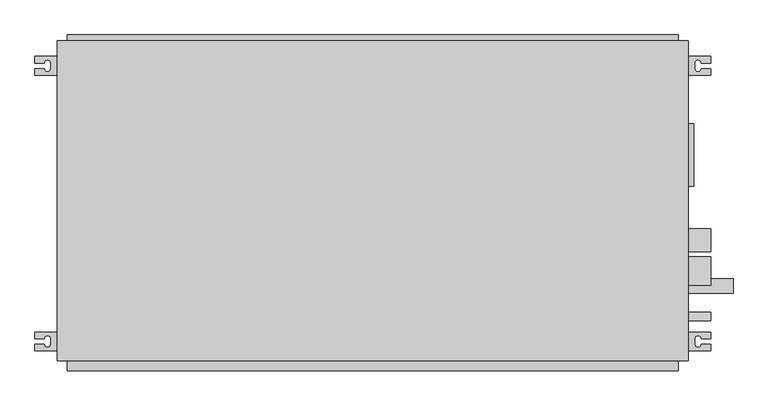
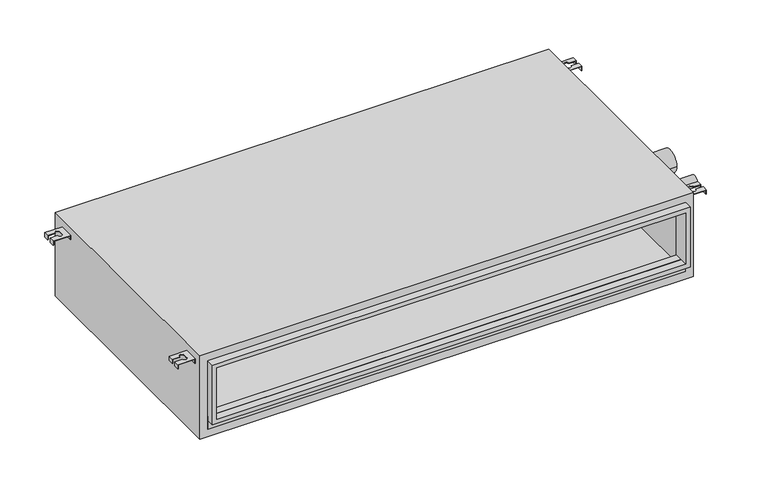
"""IFC4 building model written with IfcOpenShell, lengths in millimetres: proxy geometry, PEFY-P-NMAU-E_Medium_Static_Ducted : PEFY-P36NMAU-E."""

from ifc_helpers import new_model, si_unit, point, frame, frame_2d, origin, place, context, project, spatial, polyline, circle_curve, trimmed, segment, composite_curve, outline, extrude, source, transform, mapped, element, save
from ifc_brep_helpers import plane_surface, revolved_surface, advanced_brep


def mechanical_equipment_d478180c(model_context):
    return source(origin(), model_context, "Body", "SolidModel", [
        advanced_brep(
        [(-760.105993, -231.05, 249.2375), (-760.105993, -246.05, 249.2375), (-739.099743, -246.05, 249.2375), (-725.099743, -246.05, 249.2375), (-725.099743, -258.05, 249.2375), (-739.099743, -258.05, 249.2375), (-760.105993, -258.05, 249.2375), (-760.105993, -273.05, 249.2375), (-710.099743, -273.05, 249.2375), (-710.099743, -231.05, 249.2375), (-760.105993, -231.05, 236.4972162), (-758.517993, -231.05, 236.4972162), (-758.517993, -246.05, 236.4972162), (-760.105993, -246.05, 236.4972162), (-758.517993, -273.05, 236.4972162), (-760.105993, -273.05, 236.4972162), (-760.105993, -258.05, 236.4972162), (-758.517993, -258.05, 236.4972162), (-710.099743, -231.05, 236.4972162), (-710.099743, -273.05, 236.4972162), (-711.687743, -273.05, 236.4972162), (-711.687743, -231.05, 236.4972162), (-758.517993, -246.05, 247.65), (-739.099743, -246.05, 247.65), (-758.517993, -231.05, 247.65), (-711.687743, -231.05, 247.65), (-758.517993, -258.05, 247.65), (-758.517993, -273.05, 247.65), (-739.099743, -258.05, 247.65), (-711.687743, -273.05, 247.65), (-725.099743, -258.05, 247.65), (-725.099743, -246.05, 247.65)],
        [
            (0, 1),
            (1, 2),
            (2, 3, circle_curve(frame((-732.099743, -246.05, 249.2375), z_axis=(0.0, 0.0, -1.0), x_axis=(1.0, 0.0, 0.0)), 7.0)),
            (3, 4),
            (4, 5, circle_curve(frame((-732.099743, -258.05, 249.2375), z_axis=(0.0, 0.0, -1.0), x_axis=(1.0, 0.0, 0.0)), 7.0)),
            (5, 6),
            (6, 7),
            (7, 8),
            (8, 9),
            (9, 0),
            (10, 11),
            (11, 12),
            (12, 13),
            (13, 10),
            (14, 15),
            (15, 16),
            (16, 17),
            (17, 14),
            (18, 19),
            (19, 20),
            (20, 21),
            (21, 18),
            (13, 1),
            (0, 10),
            (12, 22),
            (22, 23),
            (23, 2),
            (11, 24),
            (24, 22),
            (9, 18),
            (21, 25),
            (25, 24),
            (17, 26),
            (26, 27),
            (27, 14),
            (5, 28),
            (28, 26),
            (16, 6),
            (15, 7),
            (27, 29),
            (29, 20),
            (19, 8),
            (29, 25),
            (30, 31),
            (31, 23, circle_curve(frame((-732.099743, -246.05, 247.65), z_axis=(0.0, 0.0, 1.0), x_axis=(1.0, 0.0, 0.0)), 7.0)),
            (28, 30, circle_curve(frame((-732.099743, -258.05, 247.65), z_axis=(0.0, 0.0, 1.0), x_axis=(1.0, 0.0, 0.0)), 7.0)),
            (4, 30),
            (31, 3),
        ],
        [
            plane_surface(frame((-760.105993, -231.05, 249.2375), z_axis=(0.0, 0.0, 1.0), x_axis=(0.0, -1.0, 0.0))),
            plane_surface(frame((-760.105993, -231.05, 236.4972162), z_axis=(0.0, 0.0, -1.0), x_axis=(0.0, 1.0, 0.0))),
            plane_surface(frame((-760.105993, -231.05, 249.2375), z_axis=(-1.0, 0.0, 0.0), x_axis=(0.0, 0.0, -1.0))),
            plane_surface(frame((-760.105993, -246.05, 249.2375), z_axis=(0.0, -1.0, 0.0), x_axis=(0.0, 0.0, -1.0))),
            plane_surface(frame((-758.517993, -246.05, 249.2375), z_axis=(1.0, 0.0, 0.0), x_axis=(0.0, 0.0, -1.0))),
            plane_surface(frame((-758.517993, -231.05, 249.2375), z_axis=(0.0, 1.0, 0.0), x_axis=(0.0, 0.0, -1.0))),
            plane_surface(frame((-758.517993, -273.05, 249.2375), z_axis=(1.0, 0.0, 0.0), x_axis=(0.0, 0.0, -1.0))),
            plane_surface(frame((-758.517993, -258.05, 249.2375), z_axis=(0.0, 1.0, 0.0), x_axis=(0.0, 0.0, -1.0))),
            plane_surface(frame((-760.105993, -258.05, 249.2375), z_axis=(-1.0, 0.0, 0.0), x_axis=(0.0, 0.0, -1.0))),
            plane_surface(frame((-760.105993, -273.05, 249.2375), z_axis=(0.0, -1.0, 0.0), x_axis=(0.0, 0.0, -1.0))),
            plane_surface(frame((-711.687743, -231.05, 249.2375), z_axis=(-1.0, 0.0, 0.0), x_axis=(0.0, 0.0, -1.0))),
            plane_surface(frame((-710.099743, -273.05, 249.2375), z_axis=(1.0, 0.0, 0.0), x_axis=(0.0, 0.0, -1.0))),
            plane_surface(frame((-725.099743, -258.05, 247.65), z_axis=(0.0, 0.0, -1.0), x_axis=(0.0, 1.0, 0.0))),
            revolved_surface(polyline([(-725.099743, -258.05, 247.65), (-725.099743, -258.05, 249.2375)]), (-732.099743, -258.05, 247.65), (0.0, 0.0, -1.0)),
            revolved_surface(polyline([(-725.099743, -246.05, 247.65), (-725.099743, -246.05, 249.2375)]), (-732.099743, -246.05, 247.65), (0.0, 0.0, -1.0)),
            plane_surface(frame((-725.099743, -246.05, 249.2375), z_axis=(-1.0, 0.0, 0.0), x_axis=(0.0, 0.0, -1.0))),
        ],
        [
            (0, [[1, 2, 3, 4, 5, 6, 7, 8, 9, 10]]),
            (1, [[11, 12, 13, 14]]),
            (1, [[15, 16, 17, 18]]),
            (1, [[19, 20, 21, 22]]),
            (2, [[23, -1, 24, -14]]),
            (3, [[-2, -23, -13, 25, 26, 27]]),
            (4, [[-12, 28, 29, -25]]),
            (5, [[-10, 30, -22, 31, 32, -28, -11, -24]]),
            (6, [[-18, 33, 34, 35]]),
            (7, [[-6, 36, 37, -33, -17, 38]]),
            (8, [[39, -7, -38, -16]]),
            (9, [[-8, -39, -15, -35, 40, 41, -20, 42]]),
            (10, [[-21, -41, 43, -31]]),
            (11, [[-30, -9, -42, -19]]),
            (12, [[44, 45, -26, -29, -32, -43, -40, -34, -37, 46]]),
            (13, [[-5, 47, -46, -36]]),
            (14, [[-3, -27, -45, 48]]),
            (15, [[-4, -48, -44, -47]]),
        ],
    ),
        advanced_brep(
        [(740.081507, -231.05, 249.2375), (690.075257, -231.05, 249.2375), (690.075257, -273.05, 249.2375), (740.081507, -273.05, 249.2375), (740.081507, -258.05, 249.2375), (719.075257, -258.05, 249.2375), (705.075257, -258.05, 249.2375), (705.075257, -246.05, 249.2375), (719.075257, -246.05, 249.2375), (740.081507, -246.05, 249.2375), (740.081507, -231.05, 236.4972162), (740.081507, -246.05, 236.4972162), (738.493507, -246.05, 236.4972162), (738.493507, -231.05, 236.4972162), (738.493507, -273.05, 236.4972162), (738.493507, -258.05, 236.4972162), (740.081507, -258.05, 236.4972162), (740.081507, -273.05, 236.4972162), (690.075257, -231.05, 236.4972162), (691.663257, -231.05, 236.4972162), (691.663257, -273.05, 236.4972162), (690.075257, -273.05, 236.4972162), (719.075257, -246.05, 247.65), (738.493507, -246.05, 247.65), (738.493507, -231.05, 247.65), (691.663257, -231.05, 247.65), (738.493507, -273.05, 247.65), (738.493507, -258.05, 247.65), (719.075257, -258.05, 247.65), (691.663257, -273.05, 247.65), (705.075257, -258.05, 247.65), (705.075257, -246.05, 247.65)],
        [
            (0, 1),
            (1, 2),
            (2, 3),
            (3, 4),
            (4, 5),
            (5, 6, circle_curve(frame((712.075257, -258.05, 249.2375), z_axis=(0.0, 0.0, -1.0), x_axis=(-1.0, 0.0, 0.0)), 7.0)),
            (6, 7),
            (7, 8, circle_curve(frame((712.075257, -246.05, 249.2375), z_axis=(0.0, 0.0, -1.0), x_axis=(-1.0, 0.0, 0.0)), 7.0)),
            (8, 9),
            (9, 0),
            (10, 11),
            (11, 12),
            (12, 13),
            (13, 10),
            (14, 15),
            (15, 16),
            (16, 17),
            (17, 14),
            (18, 19),
            (19, 20),
            (20, 21),
            (21, 18),
            (10, 0),
            (9, 11),
            (8, 22),
            (22, 23),
            (23, 12),
            (23, 24),
            (24, 13),
            (24, 25),
            (25, 19),
            (18, 1),
            (14, 26),
            (26, 27),
            (27, 15),
            (4, 16),
            (27, 28),
            (28, 5),
            (3, 17),
            (2, 21),
            (20, 29),
            (29, 26),
            (25, 29),
            (30, 28, circle_curve(frame((712.075257, -258.05, 247.65), z_axis=(0.0, 0.0, 1.0), x_axis=(-1.0, 0.0, 0.0)), 7.0)),
            (22, 31, circle_curve(frame((712.075257, -246.05, 247.65), z_axis=(0.0, 0.0, 1.0), x_axis=(-1.0, 0.0, 0.0)), 7.0)),
            (31, 30),
            (30, 6),
            (7, 31),
        ],
        [
            plane_surface(frame((740.081507, -231.05, 249.2375), z_axis=(0.0, 0.0, 1.0), x_axis=(0.0, -1.0, 0.0))),
            plane_surface(frame((740.081507, -231.05, 236.4972162), z_axis=(0.0, 0.0, -1.0), x_axis=(0.0, 1.0, 0.0))),
            plane_surface(frame((740.081507, -231.05, 249.2375), z_axis=(1.0, 0.0, 0.0), x_axis=(0.0, 0.0, -1.0))),
            plane_surface(frame((740.081507, -246.05, 249.2375), z_axis=(0.0, -1.0, 0.0), x_axis=(0.0, 0.0, -1.0))),
            plane_surface(frame((738.493507, -246.05, 249.2375), z_axis=(-1.0, 0.0, 0.0), x_axis=(0.0, 0.0, -1.0))),
            plane_surface(frame((738.493507, -231.05, 249.2375), z_axis=(0.0, 1.0, 0.0), x_axis=(0.0, 0.0, -1.0))),
            plane_surface(frame((738.493507, -273.05, 249.2375), z_axis=(-1.0, 0.0, 0.0), x_axis=(0.0, 0.0, -1.0))),
            plane_surface(frame((738.493507, -258.05, 249.2375), z_axis=(0.0, 1.0, 0.0), x_axis=(0.0, 0.0, -1.0))),
            plane_surface(frame((740.081507, -258.05, 249.2375), z_axis=(1.0, 0.0, 0.0), x_axis=(0.0, 0.0, -1.0))),
            plane_surface(frame((740.081507, -273.05, 249.2375), z_axis=(0.0, -1.0, 0.0), x_axis=(0.0, 0.0, -1.0))),
            plane_surface(frame((691.663257, -231.05, 249.2375), z_axis=(1.0, 0.0, 0.0), x_axis=(0.0, 0.0, -1.0))),
            plane_surface(frame((690.075257, -273.05, 249.2375), z_axis=(-1.0, 0.0, 0.0), x_axis=(0.0, 0.0, -1.0))),
            plane_surface(frame((705.075257, -258.05, 247.65), z_axis=(0.0, 0.0, -1.0), x_axis=(0.0, 1.0, 0.0))),
            revolved_surface(polyline([(705.075257, -258.05, 247.65), (705.075257, -258.05, 249.2375)]), (712.075257, -258.05, 247.65), (0.0, 0.0, -1.0)),
            revolved_surface(polyline([(705.075257, -246.05, 247.65), (705.075257, -246.05, 249.2375)]), (712.075257, -246.05, 247.65), (0.0, 0.0, -1.0)),
            plane_surface(frame((705.075257, -246.05, 249.2375), z_axis=(1.0, 0.0, 0.0), x_axis=(0.0, 0.0, -1.0))),
        ],
        [
            (0, [[1, 2, 3, 4, 5, 6, 7, 8, 9, 10]]),
            (1, [[11, 12, 13, 14]]),
            (1, [[15, 16, 17, 18]]),
            (1, [[19, 20, 21, 22]]),
            (2, [[-11, 23, -10, 24]]),
            (3, [[25, 26, 27, -12, -24, -9]]),
            (4, [[-27, 28, 29, -13]]),
            (5, [[-23, -14, -29, 30, 31, -19, 32, -1]]),
            (6, [[33, 34, 35, -15]]),
            (7, [[36, -16, -35, 37, 38, -5]]),
            (8, [[-17, -36, -4, 39]]),
            (9, [[40, -21, 41, 42, -33, -18, -39, -3]]),
            (10, [[-31, 43, -41, -20]]),
            (11, [[-22, -40, -2, -32]]),
            (12, [[44, -37, -34, -42, -43, -30, -28, -26, 45, 46]]),
            (13, [[-38, -44, 47, -6]]),
            (14, [[48, -45, -25, -8]]),
            (15, [[-47, -46, -48, -7]]),
        ],
    ),
        advanced_brep(
        [(-760.105993, 339.0, 249.2375), (-710.099743, 339.0, 249.2375), (-710.099743, 381.0, 249.2375), (-760.105993, 381.0, 249.2375), (-760.105993, 366.0, 249.2375), (-739.099743, 366.0, 249.2375), (-725.099743, 366.0, 249.2375), (-725.099743, 354.0, 249.2375), (-739.099743, 354.0, 249.2375), (-760.105993, 354.0, 249.2375), (-760.105993, 339.0, 236.4972162), (-760.105993, 354.0, 236.4972162), (-758.517993, 354.0, 236.4972162), (-758.517993, 339.0, 236.4972162), (-758.517993, 381.0, 236.4972162), (-758.517993, 366.0, 236.4972162), (-760.105993, 366.0, 236.4972162), (-760.105993, 381.0, 236.4972162), (-710.099743, 339.0, 236.4972162), (-711.687743, 339.0, 236.4972162), (-711.687743, 381.0, 236.4972162), (-710.099743, 381.0, 236.4972162), (-739.099743, 354.0, 247.65), (-758.517993, 354.0, 247.65), (-758.517993, 339.0, 247.65), (-711.687743, 339.0, 247.65), (-758.517993, 381.0, 247.65), (-758.517993, 366.0, 247.65), (-739.099743, 366.0, 247.65), (-711.687743, 381.0, 247.65), (-725.099743, 366.0, 247.65), (-725.099743, 354.0, 247.65)],
        [
            (0, 1),
            (1, 2),
            (2, 3),
            (3, 4),
            (4, 5),
            (5, 6, circle_curve(frame((-732.099743, 366.0, 249.2375), z_axis=(0.0, 0.0, -1.0), x_axis=(1.0, 0.0, 0.0)), 7.0)),
            (6, 7),
            (7, 8, circle_curve(frame((-732.099743, 354.0, 249.2375), z_axis=(0.0, 0.0, -1.0), x_axis=(1.0, 0.0, 0.0)), 7.0)),
            (8, 9),
            (9, 0),
            (10, 11),
            (11, 12),
            (12, 13),
            (13, 10),
            (14, 15),
            (15, 16),
            (16, 17),
            (17, 14),
            (18, 19),
            (19, 20),
            (20, 21),
            (21, 18),
            (10, 0),
            (9, 11),
            (8, 22),
            (22, 23),
            (23, 12),
            (23, 24),
            (24, 13),
            (24, 25),
            (25, 19),
            (18, 1),
            (14, 26),
            (26, 27),
            (27, 15),
            (4, 16),
            (27, 28),
            (28, 5),
            (3, 17),
            (2, 21),
            (20, 29),
            (29, 26),
            (25, 29),
            (30, 28, circle_curve(frame((-732.099743, 366.0, 247.65), z_axis=(0.0, 0.0, 1.0), x_axis=(1.0, 0.0, 0.0)), 7.0)),
            (22, 31, circle_curve(frame((-732.099743, 354.0, 247.65), z_axis=(0.0, 0.0, 1.0), x_axis=(1.0, 0.0, 0.0)), 7.0)),
            (31, 30),
            (30, 6),
            (7, 31),
        ],
        [
            plane_surface(frame((-760.105993, 339.0, 249.2375), z_axis=(0.0, 0.0, 1.0), x_axis=(0.0, 1.0, 0.0))),
            plane_surface(frame((-760.105993, 339.0, 236.4972162), z_axis=(0.0, 0.0, -1.0), x_axis=(0.0, -1.0, 0.0))),
            plane_surface(frame((-760.105993, 339.0, 249.2375), z_axis=(-1.0, 0.0, 0.0), x_axis=(0.0, 0.0, -1.0))),
            plane_surface(frame((-760.105993, 354.0, 249.2375), z_axis=(0.0, 1.0, 0.0), x_axis=(0.0, 0.0, -1.0))),
            plane_surface(frame((-758.517993, 354.0, 249.2375), z_axis=(1.0, 0.0, 0.0), x_axis=(0.0, 0.0, -1.0))),
            plane_surface(frame((-758.517993, 339.0, 249.2375), z_axis=(0.0, -1.0, 0.0), x_axis=(0.0, 0.0, -1.0))),
            plane_surface(frame((-758.517993, 381.0, 249.2375), z_axis=(1.0, 0.0, 0.0), x_axis=(0.0, 0.0, -1.0))),
            plane_surface(frame((-758.517993, 366.0, 249.2375), z_axis=(0.0, -1.0, 0.0), x_axis=(0.0, 0.0, -1.0))),
            plane_surface(frame((-760.105993, 366.0, 249.2375), z_axis=(-1.0, 0.0, 0.0), x_axis=(0.0, 0.0, -1.0))),
            plane_surface(frame((-760.105993, 381.0, 249.2375), z_axis=(0.0, 1.0, 0.0), x_axis=(0.0, 0.0, -1.0))),
            plane_surface(frame((-711.687743, 339.0, 249.2375), z_axis=(-1.0, 0.0, 0.0), x_axis=(0.0, 0.0, -1.0))),
            plane_surface(frame((-710.099743, 381.0, 249.2375), z_axis=(1.0, 0.0, 0.0), x_axis=(0.0, 0.0, -1.0))),
            plane_surface(frame((-725.099743, 366.0, 247.65), z_axis=(0.0, 0.0, -1.0), x_axis=(0.0, -1.0, 0.0))),
            revolved_surface(polyline([(-725.099743, 366.0, 247.65), (-725.099743, 366.0, 249.2375)]), (-732.099743, 366.0, 247.65), (0.0, 0.0, -1.0)),
            revolved_surface(polyline([(-725.099743, 354.0, 247.65), (-725.099743, 354.0, 249.2375)]), (-732.099743, 354.0, 247.65), (0.0, 0.0, -1.0)),
            plane_surface(frame((-725.099743, 354.0, 249.2375), z_axis=(-1.0, 0.0, 0.0), x_axis=(0.0, 0.0, -1.0))),
        ],
        [
            (0, [[1, 2, 3, 4, 5, 6, 7, 8, 9, 10]]),
            (1, [[11, 12, 13, 14]]),
            (1, [[15, 16, 17, 18]]),
            (1, [[19, 20, 21, 22]]),
            (2, [[-11, 23, -10, 24]]),
            (3, [[25, 26, 27, -12, -24, -9]]),
            (4, [[-27, 28, 29, -13]]),
            (5, [[-23, -14, -29, 30, 31, -19, 32, -1]]),
            (6, [[33, 34, 35, -15]]),
            (7, [[36, -16, -35, 37, 38, -5]]),
            (8, [[-17, -36, -4, 39]]),
            (9, [[40, -21, 41, 42, -33, -18, -39, -3]]),
            (10, [[-31, 43, -41, -20]]),
            (11, [[-22, -40, -2, -32]]),
            (12, [[44, -37, -34, -42, -43, -30, -28, -26, 45, 46]]),
            (13, [[-38, -44, 47, -6]]),
            (14, [[48, -45, -25, -8]]),
            (15, [[-47, -46, -48, -7]]),
        ],
    ),
        advanced_brep(
        [(740.081507, 339.0, 249.2375), (740.081507, 354.0, 249.2375), (719.075257, 354.0, 249.2375), (705.075257, 354.0, 249.2375), (705.075257, 366.0, 249.2375), (719.075257, 366.0, 249.2375), (740.081507, 366.0, 249.2375), (740.081507, 381.0, 249.2375), (690.075257, 381.0, 249.2375), (690.075257, 339.0, 249.2375), (740.081507, 339.0, 236.4972162), (738.493507, 339.0, 236.4972162), (738.493507, 354.0, 236.4972162), (740.081507, 354.0, 236.4972162), (738.493507, 381.0, 236.4972162), (740.081507, 381.0, 236.4972162), (740.081507, 366.0, 236.4972162), (738.493507, 366.0, 236.4972162), (690.075257, 339.0, 236.4972162), (690.075257, 381.0, 236.4972162), (691.663257, 381.0, 236.4972162), (691.663257, 339.0, 236.4972162), (738.493507, 354.0, 247.65), (719.075257, 354.0, 247.65), (738.493507, 339.0, 247.65), (691.663257, 339.0, 247.65), (738.493507, 366.0, 247.65), (738.493507, 381.0, 247.65), (719.075257, 366.0, 247.65), (691.663257, 381.0, 247.65), (705.075257, 366.0, 247.65), (705.075257, 354.0, 247.65)],
        [
            (0, 1),
            (1, 2),
            (2, 3, circle_curve(frame((712.075257, 354.0, 249.2375), z_axis=(0.0, 0.0, -1.0), x_axis=(-1.0, 0.0, 0.0)), 7.0)),
            (3, 4),
            (4, 5, circle_curve(frame((712.075257, 366.0, 249.2375), z_axis=(0.0, 0.0, -1.0), x_axis=(-1.0, 0.0, 0.0)), 7.0)),
            (5, 6),
            (6, 7),
            (7, 8),
            (8, 9),
            (9, 0),
            (10, 11),
            (11, 12),
            (12, 13),
            (13, 10),
            (14, 15),
            (15, 16),
            (16, 17),
            (17, 14),
            (18, 19),
            (19, 20),
            (20, 21),
            (21, 18),
            (13, 1),
            (0, 10),
            (12, 22),
            (22, 23),
            (23, 2),
            (11, 24),
            (24, 22),
            (9, 18),
            (21, 25),
            (25, 24),
            (17, 26),
            (26, 27),
            (27, 14),
            (5, 28),
            (28, 26),
            (16, 6),
            (15, 7),
            (27, 29),
            (29, 20),
            (19, 8),
            (29, 25),
            (30, 31),
            (31, 23, circle_curve(frame((712.075257, 354.0, 247.65), z_axis=(0.0, 0.0, 1.0), x_axis=(-1.0, 0.0, 0.0)), 7.0)),
            (28, 30, circle_curve(frame((712.075257, 366.0, 247.65), z_axis=(0.0, 0.0, 1.0), x_axis=(-1.0, 0.0, 0.0)), 7.0)),
            (4, 30),
            (31, 3),
        ],
        [
            plane_surface(frame((740.081507, 339.0, 249.2375), z_axis=(0.0, 0.0, 1.0), x_axis=(0.0, 1.0, 0.0))),
            plane_surface(frame((740.081507, 339.0, 236.4972162), z_axis=(0.0, 0.0, -1.0), x_axis=(0.0, -1.0, 0.0))),
            plane_surface(frame((740.081507, 339.0, 249.2375), z_axis=(1.0, 0.0, 0.0), x_axis=(0.0, 0.0, -1.0))),
            plane_surface(frame((740.081507, 354.0, 249.2375), z_axis=(0.0, 1.0, 0.0), x_axis=(0.0, 0.0, -1.0))),
            plane_surface(frame((738.493507, 354.0, 249.2375), z_axis=(-1.0, 0.0, 0.0), x_axis=(0.0, 0.0, -1.0))),
            plane_surface(frame((738.493507, 339.0, 249.2375), z_axis=(0.0, -1.0, 0.0), x_axis=(0.0, 0.0, -1.0))),
            plane_surface(frame((738.493507, 381.0, 249.2375), z_axis=(-1.0, 0.0, 0.0), x_axis=(0.0, 0.0, -1.0))),
            plane_surface(frame((738.493507, 366.0, 249.2375), z_axis=(0.0, -1.0, 0.0), x_axis=(0.0, 0.0, -1.0))),
            plane_surface(frame((740.081507, 366.0, 249.2375), z_axis=(1.0, 0.0, 0.0), x_axis=(0.0, 0.0, -1.0))),
            plane_surface(frame((740.081507, 381.0, 249.2375), z_axis=(0.0, 1.0, 0.0), x_axis=(0.0, 0.0, -1.0))),
            plane_surface(frame((691.663257, 339.0, 249.2375), z_axis=(1.0, 0.0, 0.0), x_axis=(0.0, 0.0, -1.0))),
            plane_surface(frame((690.075257, 381.0, 249.2375), z_axis=(-1.0, 0.0, 0.0), x_axis=(0.0, 0.0, -1.0))),
            plane_surface(frame((705.075257, 366.0, 247.65), z_axis=(0.0, 0.0, -1.0), x_axis=(0.0, -1.0, 0.0))),
            revolved_surface(polyline([(705.075257, 366.0, 247.65), (705.075257, 366.0, 249.2375)]), (712.075257, 366.0, 247.65), (0.0, 0.0, -1.0)),
            revolved_surface(polyline([(705.075257, 354.0, 247.65), (705.075257, 354.0, 249.2375)]), (712.075257, 354.0, 247.65), (0.0, 0.0, -1.0)),
            plane_surface(frame((705.075257, 354.0, 249.2375), z_axis=(1.0, 0.0, 0.0), x_axis=(0.0, 0.0, -1.0))),
        ],
        [
            (0, [[1, 2, 3, 4, 5, 6, 7, 8, 9, 10]]),
            (1, [[11, 12, 13, 14]]),
            (1, [[15, 16, 17, 18]]),
            (1, [[19, 20, 21, 22]]),
            (2, [[23, -1, 24, -14]]),
            (3, [[-2, -23, -13, 25, 26, 27]]),
            (4, [[-12, 28, 29, -25]]),
            (5, [[-10, 30, -22, 31, 32, -28, -11, -24]]),
            (6, [[-18, 33, 34, 35]]),
            (7, [[-6, 36, 37, -33, -17, 38]]),
            (8, [[39, -7, -38, -16]]),
            (9, [[-8, -39, -15, -35, 40, 41, -20, 42]]),
            (10, [[-21, -41, 43, -31]]),
            (11, [[-30, -9, -42, -19]]),
            (12, [[44, 45, -26, -29, -32, -43, -40, -34, -37, 46]]),
            (13, [[-5, 47, -46, -36]]),
            (14, [[-3, -27, -45, 48]]),
            (15, [[-4, -48, -44, -47]]),
        ],
    ),
        extrude(outline(polyline([(667.850257, -295.275), (-687.874743, -295.275), (-687.874743, -273.05), (667.850257, -273.05), (667.850257, -295.275)])), frame((0.0, 0.0, 42.8625), z_axis=(0.0, 0.0, 1.0), x_axis=(1.0, 0.0, 0.0)), (0.0, 0.0, 1.0), 39.6875),
        extrude(outline(polyline([(249.2375, 667.850257), (249.2375, -687.874743), (69.85, -687.874743), (69.85, 667.850257), (249.2375, 667.850257)]), holes=[polyline([(82.55, 655.150257), (82.55, -675.174743), (236.5375, -675.174743), (236.5375, 655.150257), (82.55, 655.150257)])]), frame((0.0, -317.5, 0.0), z_axis=(0.0, 1.0, 0.0), x_axis=(0.0, 0.0, 1.0)), (0.0, 0.0, 1.0), 44.45),
        extrude(outline(polyline([(667.850257, 415.925), (-687.874743, 415.925), (-687.874743, 428.625), (667.850257, 428.625), (667.850257, 415.925)])), frame((0.0, 0.0, 42.8625), z_axis=(0.0, 0.0, 1.0), x_axis=(1.0, 0.0, 0.0)), (0.0, 0.0, 1.0), 206.375),
        extrude(outline(polyline([(271.4625, 690.075257), (271.4625, -710.099743), (20.6375, -710.099743), (20.6375, 690.075257), (271.4625, 690.075257)]), holes=[polyline([(42.8625, -687.874743), (249.2375, -687.874743), (249.2375, 667.850257), (42.8625, 667.850257), (42.8625, -687.874743)])]), frame((0.0, -295.275, 0.0), z_axis=(0.0, 1.0, 0.0), x_axis=(0.0, 0.0, 1.0)), (0.0, 0.0, 1.0), 711.2),
        extrude(outline(composite_curve([segment(trimmed(circle_curve(frame_2d((-26.9875, 109.5375)), 25.4), [point((-1.5875, 109.5375))], [point((-52.3875, 109.5375))], False, "CARTESIAN"), True, "CONTINUOUS"), segment(trimmed(circle_curve(frame_2d((-26.9875, 109.5375)), 25.4), [point((-52.3875, 109.5375))], [point((-1.5875, 109.5375))], False, "CARTESIAN"), True, "CONTINUOUS")], self_intersect=False)), frame((690.075257, 0.0, 0.0), z_axis=(1.0, 0.0, 0.0), x_axis=(0.0, 1.0, 0.0)), (0.0, 0.0, 1.0), 50.00625),
        extrude(outline(composite_curve([segment(trimmed(circle_curve(frame_2d((-128.5875, 171.45)), 15.875), [point((-112.7125, 171.45))], [point((-144.4625, 171.45))], False, "CARTESIAN"), True, "CONTINUOUS"), segment(trimmed(circle_curve(frame_2d((-128.5875, 171.45)), 15.875), [point((-144.4625, 171.45))], [point((-112.7125, 171.45))], False, "CARTESIAN"), True, "CONTINUOUS")], self_intersect=False)), frame((690.075257, 0.0, 0.0), z_axis=(1.0, 0.0, 0.0), x_axis=(0.0, 1.0, 0.0)), (0.0, 0.0, 1.0), 100.0125),
        extrude(outline(composite_curve([segment(trimmed(circle_curve(frame_2d((-95.25, 230.1875)), 31.75), [point((-63.5, 230.1875))], [point((-127.0, 230.1875))], False, "CARTESIAN"), True, "CONTINUOUS"), segment(trimmed(circle_curve(frame_2d((-95.25, 230.1875)), 31.75), [point((-127.0, 230.1875))], [point((-63.5, 230.1875))], False, "CARTESIAN"), True, "CONTINUOUS")], self_intersect=False)), frame((690.075257, 0.0, 0.0), z_axis=(1.0, 0.0, 0.0), x_axis=(0.0, 1.0, 0.0)), (0.0, 0.0, 1.0), 50.00625),
        extrude(outline(composite_curve([segment(trimmed(circle_curve(frame_2d((-196.85, 104.775)), 9.525), [point((-187.325, 104.775))], [point((-206.375, 104.775))], False, "CARTESIAN"), True, "CONTINUOUS"), segment(trimmed(circle_curve(frame_2d((-196.85, 104.775)), 9.525), [point((-206.375, 104.775))], [point((-187.325, 104.775))], False, "CARTESIAN"), True, "CONTINUOUS")], self_intersect=False)), frame((690.075257, 0.0, 0.0), z_axis=(1.0, 0.0, 0.0), x_axis=(0.0, 1.0, 0.0)), (0.0, 0.0, 1.0), 50.00625),
        extrude(outline(polyline([(702.775257, 231.84375), (702.775257, 92.14375), (690.075257, 92.14375), (690.075257, 231.84375), (702.775257, 231.84375)])), frame((0.0, 0.0, 42.8625), z_axis=(0.0, 0.0, 1.0), x_axis=(1.0, 0.0, 0.0)), (0.0, 0.0, 1.0), 187.325),
    ])


if __name__ == "__main__":
    model = new_model("IFC4")
    model_context = context("Model", 3, world=origin())
    ifc_project = project(units=[si_unit("LENGTHUNIT", "METRE", prefix="MILLI")], contexts=[model_context])
    site = spatial("IfcSite", under=ifc_project)
    building = spatial("IfcBuilding", under=site)
    placement = place(None, origin())
    mechanical_equipment_shape = mechanical_equipment_d478180c(model_context)
    element("IfcBuildingElementProxy", 1, Name="PEFY-P-NMAU-E_Medium_Static_Ducted : PEFY-P36NMAU-E", ObjectType="PEFY-P-NMAU-E_Medium_Static_Ducted : PEFY-P36NMAU-E", at=placement, inside=building, context=model_context, shape_type="MappedRepresentation", body=[
        mapped(mechanical_equipment_shape, transform((0.0, 0.0, 0.0), x_axis=(1.0, 0.0, 0.0), y_axis=(0.0, 1.0, 0.0), z_axis=(0.0, 0.0, 1.0))),
    ])
    save(model, "model.ifc")

# Revit data of these elements
# Type "PEFY-P-NMAU-E_Medium_Static_Ducted : PEFY-P36NMAU-E"
#   Wiring (Min.size of wire) = "1/8"
#   Wiring (Amperage of wire breaker) = "15 A"
#   Voltage Options = "208/230 VAC"
#   Unit Weight (LBS) = "93"
#   Temperature set range Remote controller Heating = "63 to 83 F"
#   Temperature set range Remote controller Cooling = "67 to 86 F"
#   Subcategory = "HVAC"
#   Specification URL = ""
#   Sound Pressure Levels (dB(A)) = "26,28,29"
#   SmartBIM Object Created By = "Reed Construction Data"
#   Single Phase = "X"
#   Refrigerant control device = "LEV"
#   Protection devices = "Fuse"
#   Power input Heating = "0.22 kW"
#   Power input Cooling = "0.24 kW"
#   Moter Type = "DC blushless motor"
#   Moter Output = "0.085 kW"
#   Model = "PEFY-P36NMAU-E"
#   Manufacturer URL = ""
#   Manufacturer = "Mitsubishi Electric"
#   Insulation material = "EPS, Polyethylene foam, Urethane foam"
#   Installation URL = ""
#   Heating Capacity (kcal/h) = "10,100"
#   Heating Capacity (kW) = "11.7"
#   Heat exchanger = "Cross fin(Aluminium fin and copper tube)"
#   Frequency = "60 Hz"
#   Fan Type x Quantity = "Sirocco fan x 1"
#   E.S.P(mmH2O) = "3.6,5.1,7.1,10.2,15.3"
#   E.S.P(Pa) = "35,50,70,100,150"
#   E.S.P(In. W.G.) = "0.14,0.20,0.28,0.40,0.60"
#   Driving mechanism = "Direct-driven by motor"
#   Current Heating = "1.39 A"
#   Current Cooling = "1.50 A"
#   Cooling Capacity (kcal/h) = "9,100"
#   Cooling Capacity (kW) = "10.6"
#   Connectable outdoor unit = "R410A,R22 CITY MULTI"
#   Assembly Code = "D3050200"
#   Airflow rate(Low-Mid-High) (m3/min) = "6.0,7.5,8.5"
#   Airflow rate(Low-Mid-High) (cfm) = "212,265,300"
#   Airflow rate(Low-Mid-High) (L/s) = "100,125,142"
#   Air Filter = "PP Honeycomb fabric"
#   95 CSI = "15760"
#   04 CSI = "23 82 19"
#   Width = 1400.175 mm
#   Voltage = 208 V
#   Unit Supply Airflow [instance default] = 0 CFM
#   Unit Return Airflow [instance default] = 0 CFM
#   SmartBIM Object Version = 3
#   Refrigerant Pipe Liquid = 9.525 mm
#   Refrigerant Pipe Gas = 15.875 mm
#   Refirigerant Pipe diameter (Liquid) = 9.525 mm
#   Refirigerant Pipe diameter (Gas) = 15.875 mm
#   Phase = 1
#   Nominal Heating Capacity = 40000.0 Btu/h
#   Nominal Cooling Capacity = 36000.0 Btu/h
#   Minimum Circuit Current = 3.33 A
#   Maximum Overcurrent Protection = 15 A
#   Hertz = 60
#   Height = 250.825 mm
#   Drain piping diameter = 31.75 mm
#   Drain Pump = 25.4 mm
#   Depth = 733.425 mm
#   Default Elevation = 1219.2 mm
#   Back Air Inlet Width = 1355.725 mm
#   Back Air Inlet Height = 206.375 mm
#   Apparent Load = 0 VA
#   Air Outlet Width = 1355.725 mm
#   Air Outlet Height = 179.388 mm
#   Sound Pressure Levels @ Mid Airflow (dBA) = 37
#   Sound Pressure Levels @ Low Airflow (dBA) = 32
#   Sound Pressure Levels @ High Airflow (dBA) = 41
#   Number of Poles = 2
#   Unit = Metal - Steel Satin
#   Load Classification = Other
#   Back Air Inlet = Grille
# Element 1 (IfcBuildingElementProxy, "PEFY-P-NMAU-E_Medium_Static_Ducted : PEFY-P36NMAU-E")
#   Unit Supply Airflow = 1060 CFM
#   Unit Return Airflow = 1060 CFM
#   Materials on its faces: "Metal - Steel Satin", "Grille"
# Materials
#   "Metal - Steel Satin": class "Metal", colour RGB 189 187 185, transparency 0
#   "Grille": class "Miscellaneous", colour RGB 0 0 0, transparency 0
